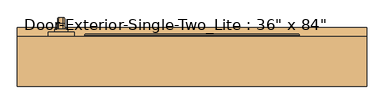
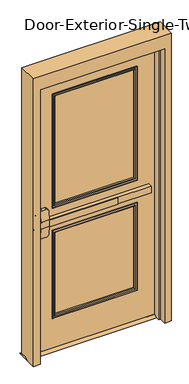
"""IFC4 building model written with IfcOpenShell, lengths in millimetres: door geometry."""

from ifc_helpers import new_model, si_unit, point, frame, frame_2d, origin, place, context, project, spatial, polyline, circle_curve, ellipse_curve, trimmed, segment, composite_curve, outline, extrude, faceted_brep, source, transform, mapped, element, save
from ifc_brep_helpers import plane_surface, cylinder_surface, revolved_surface, advanced_brep


def door_1117bd37(model_context):
    return source(origin(), model_context, "Body", "SolidModel", [
        extrude(outline(polyline([(76.2, 12.7), (120.65, 12.7), (146.05, 0.0), (50.8, 0.0), (76.2, 12.7)])), frame((-508.0, 0.0, 0.0), z_axis=(1.0, 0.0, 0.0), x_axis=(0.0, 1.0, 0.0)), (0.0, 0.0, 1.0), 1016.0),
        extrude(outline(polyline([(150.2833333, 38.1), (-349.25, 38.1), (-349.25, 44.45), (150.2833333, 44.45), (150.2833333, 38.1)])), frame((0.0, 0.0, 990.6), z_axis=(0.0, 0.0, 1.0), x_axis=(1.0, 0.0, 0.0)), (0.0, 0.0, 1.0), 50.8),
        advanced_brep(
        [(-412.75, 44.45, 1041.4), (-412.75, 44.45, 990.6), (-349.25, 44.45, 990.6), (400.05, 44.45, 990.6), (400.05, 44.45, 1041.4), (-349.25, 44.45, 1041.4), (400.05, 76.2, 1041.4), (400.05, 76.2, 990.6), (-349.25, 76.2, 990.6), (-349.25, 76.2, 927.1), (-368.3, 76.2, 908.05), (-393.7, 76.2, 908.05), (-412.75, 76.2, 927.1), (-412.75, 76.2, 1104.9), (-393.7, 76.2, 1123.95), (-368.3, 76.2, 1123.95), (-349.25, 76.2, 1104.9), (-349.25, 76.2, 1041.4), (-349.25, 47.6252467, 1041.4), (-412.75, 47.6252467, 1041.4), (-412.75, 52.6354269, 1104.9), (-412.75, 52.6354269, 927.1), (-412.75, 47.6252467, 990.6), (-349.25, 47.6252467, 990.6), (-349.25, 52.6354269, 927.1), (-349.25, 52.6354269, 1104.9), (-393.7, 54.138481, 1123.95), (-368.3, 54.138481, 1123.95), (-368.3, 54.138481, 908.05), (-393.7, 54.138481, 908.05)],
        [
            (0, 1),
            (1, 2),
            (2, 3),
            (3, 4),
            (4, 5),
            (5, 0),
            (6, 7),
            (7, 8),
            (8, 9),
            (9, 10, circle_curve(frame((-368.3, 76.2, 927.1), z_axis=(0.0, 1.0, 0.0), x_axis=(1.0, 0.0, 0.0)), 19.05)),
            (10, 11),
            (11, 12, circle_curve(frame((-393.7, 76.2, 927.1), z_axis=(0.0, 1.0, 0.0), x_axis=(1.0, 0.0, 0.0)), 19.05)),
            (12, 13),
            (13, 14, circle_curve(frame((-393.7, 76.2, 1104.9), z_axis=(0.0, 1.0, 0.0), x_axis=(1.0, 0.0, 0.0)), 19.05)),
            (14, 15),
            (15, 16, circle_curve(frame((-368.3, 76.2, 1104.9), z_axis=(0.0, 1.0, 0.0), x_axis=(1.0, 0.0, 0.0)), 19.05)),
            (16, 17),
            (17, 6),
            (4, 6),
            (17, 18),
            (18, 19),
            (19, 0),
            (19, 20),
            (20, 13),
            (12, 21),
            (21, 22),
            (22, 1),
            (7, 3),
            (22, 23),
            (23, 8),
            (23, 24),
            (24, 9),
            (16, 25),
            (25, 18),
            (14, 26),
            (26, 27),
            (27, 15),
            (10, 28),
            (28, 29),
            (29, 11),
            (24, 28, ellipse_curve(frame((-368.3, 52.6354269, 927.1), z_axis=(0.0, 0.9969018152893365, 0.07865602756830282), x_axis=(0.0, -0.07865602756830208, 0.9969018152893365)), 19.1092038, 19.05)),
            (27, 25, ellipse_curve(frame((-368.3, 52.6354269, 1104.9), z_axis=(0.0, 0.9969018152893376, -0.07865602756828934), x_axis=(0.0, -0.078656027568288, -0.9969018152893377)), 19.1092038, 19.05)),
            (20, 26, ellipse_curve(frame((-393.7, 52.6354269, 1104.9), z_axis=(0.0, 0.9969018152893376, -0.07865602756828934), x_axis=(0.0, -0.078656027568288, -0.9969018152893377)), 19.1092038, 19.05)),
            (29, 21, ellipse_curve(frame((-393.7, 52.6354269, 927.1), z_axis=(0.0, 0.9969018152893365, 0.07865602756830282), x_axis=(0.0, -0.07865602756830208, 0.9969018152893365)), 19.1092038, 19.05)),
        ],
        [
            plane_surface(frame((-412.75, 44.45, 1041.4), z_axis=(0.0, -1.0, 0.0), x_axis=(-1.0, 0.0, 0.0))),
            plane_surface(frame((-412.75, 76.2, 1041.4), z_axis=(0.0, 1.0, 0.0), x_axis=(1.0, 0.0, 0.0))),
            plane_surface(frame((400.05, 44.45, 1041.4), z_axis=(0.0, 0.0, 1.0), x_axis=(0.0, 1.0, 0.0))),
            plane_surface(frame((-412.75, 44.45, 1041.4), z_axis=(-1.0, 0.0, 0.0), x_axis=(0.0, 1.0, 0.0))),
            plane_surface(frame((-412.75, 44.45, 990.6), z_axis=(0.0, 0.0, -1.0), x_axis=(0.0, 1.0, 0.0))),
            plane_surface(frame((400.05, 44.45, 990.6), z_axis=(1.0, 0.0, 0.0), x_axis=(0.0, 1.0, 0.0))),
            plane_surface(frame((-349.25, 47.6252467, 927.1), z_axis=(1.0, 0.0, 0.0), x_axis=(0.0, 1.0, 0.0))),
            plane_surface(frame((-368.3, 47.6252467, 1123.95), z_axis=(0.0, 0.0, 1.0), x_axis=(0.0, 1.0, 0.0))),
            plane_surface(frame((-393.7, 47.6252467, 908.05), z_axis=(0.0, 0.0, -1.0), x_axis=(0.0, 1.0, 0.0))),
            cylinder_surface(frame((-368.3, 76.2, 927.1), z_axis=(0.0, -1.0, 0.0), x_axis=(1.0, 0.0, 0.0)), 19.05),
            cylinder_surface(frame((-368.3, 76.2, 1104.9), z_axis=(0.0, -1.0, 0.0), x_axis=(1.0, 0.0, 0.0)), 19.05),
            cylinder_surface(frame((-393.7, 76.2, 1104.9), z_axis=(0.0, -1.0, 0.0), x_axis=(1.0, 0.0, 0.0)), 19.05),
            cylinder_surface(frame((-393.7, 76.2, 927.1), z_axis=(0.0, -1.0, 0.0), x_axis=(1.0, 0.0, 0.0)), 19.05),
            plane_surface(frame((-349.25, 47.6252467, 1041.4), z_axis=(0.0, -0.9969018152893376, 0.07865602756828934), x_axis=(-1.0, 0.0, 0.0))),
            plane_surface(frame((-349.25, 54.138481, 908.05), z_axis=(0.0, -0.9969018152893365, -0.07865602756830282), x_axis=(-1.0, 0.0, 0.0))),
        ],
        [
            (0, [[1, 2, 3, 4, 5, 6]]),
            (1, [[7, 8, 9, 10, 11, 12, 13, 14, 15, 16, 17, 18]]),
            (2, [[19, -18, 20, 21, 22, -6, -5]]),
            (3, [[-1, -22, 23, 24, -13, 25, 26, 27]]),
            (4, [[28, -3, -2, -27, 29, 30, -8]]),
            (5, [[-4, -28, -7, -19]]),
            (6, [[-9, -30, 31, 32]]),
            (6, [[-17, 33, 34, -20]]),
            (7, [[-15, 35, 36, 37]]),
            (8, [[-11, 38, 39, 40]]),
            (9, [[-10, -32, 41, -38]]),
            (10, [[-16, -37, 42, -33]]),
            (11, [[-14, -24, 43, -35]]),
            (12, [[-12, -40, 44, -25]]),
            (13, [[-21, -34, -42, -36, -43, -23]]),
            (14, [[-26, -44, -39, -41, -31, -29]]),
        ],
    ),
        advanced_brep(
        [(-391.0, 133.35, 1017.190625), (-391.0, 133.35, 1014.809375), (-387.428125, 133.35, 1011.2375), (-374.5715406, 133.35, 1011.2375), (-371.0, 133.35, 1014.8090406), (-371.0, 133.35, 1017.190625), (-374.571875, 133.35, 1020.7625), (-387.428125, 133.35, 1020.7625), (-391.0, 133.35, 887.809375), (-387.428125, 133.35, 884.2375), (-374.571875, 133.35, 884.2375), (-371.0, 133.35, 887.809375), (-371.0, 133.35, 890.1909594), (-374.5715406, 133.35, 893.7625), (-387.428125, 133.35, 893.7625), (-391.0, 133.35, 890.190625), (-391.0, 158.75, 1017.190625), (-391.0, 172.640625, 1003.3), (-391.0, 172.640625, 901.7), (-391.0, 158.75, 887.809375), (-391.0, 158.75, 890.190625), (-391.0, 170.259375, 901.7), (-391.0, 170.259375, 1003.3), (-391.0, 158.75, 1014.809375), (-387.428125, 158.75, 1011.2375), (-374.5715406, 158.75, 1011.2375), (-371.0, 158.75, 1014.8090406), (-371.0, 170.2590406, 1003.3), (-371.0, 170.2590406, 901.7), (-371.0, 158.75, 890.1909594), (-371.0, 158.75, 887.809375), (-371.0, 172.640625, 901.7), (-371.0, 172.640625, 1003.3), (-371.0, 158.75, 1017.190625), (-374.571875, 158.75, 1020.7625), (-387.428125, 158.75, 1020.7625), (-387.428125, 166.6875, 1003.3), (-374.5715406, 166.6875, 1003.3), (-374.571875, 176.2125, 1003.3), (-387.428125, 176.2125, 1003.3), (-387.428125, 166.6875, 901.7), (-374.5715406, 166.6875, 901.7), (-374.571875, 176.2125, 901.7), (-387.428125, 176.2125, 901.7), (-387.428125, 158.75, 893.7625), (-374.5715406, 158.75, 893.7625), (-374.571875, 158.75, 884.2375), (-387.428125, 158.75, 884.2375)],
        [
            (0, 1),
            (1, 2, circle_curve(frame((-387.428125, 133.35, 1014.809375), z_axis=(0.0, -1.0, 0.0), x_axis=(0.0, 0.0, 1.0)), 3.571875)),
            (2, 3),
            (3, 4, circle_curve(frame((-374.5715406, 133.35, 1014.8090406), z_axis=(0.0, -1.0, 0.0), x_axis=(0.0, 0.0, 1.0)), 3.5715406)),
            (4, 5),
            (5, 6, circle_curve(frame((-374.571875, 133.35, 1017.190625), z_axis=(0.0, -1.0, 0.0), x_axis=(0.0, 0.0, 1.0)), 3.571875)),
            (6, 7),
            (7, 0, circle_curve(frame((-387.428125, 133.35, 1017.190625), z_axis=(0.0, -1.0, 0.0), x_axis=(0.0, 0.0, 1.0)), 3.571875)),
            (8, 9, circle_curve(frame((-387.428125, 133.35, 887.809375), z_axis=(0.0, -1.0, 0.0), x_axis=(0.0, 0.0, -1.0)), 3.571875)),
            (9, 10),
            (10, 11, circle_curve(frame((-374.571875, 133.35, 887.809375), z_axis=(0.0, -1.0, 0.0), x_axis=(0.0, 0.0, -1.0)), 3.571875)),
            (11, 12),
            (12, 13, circle_curve(frame((-374.5715406, 133.35, 890.1909594), z_axis=(0.0, -1.0, 0.0), x_axis=(0.0, 0.0, -1.0)), 3.5715406)),
            (13, 14),
            (14, 15, circle_curve(frame((-387.428125, 133.35, 890.190625), z_axis=(0.0, -1.0, 0.0), x_axis=(0.0, 0.0, -1.0)), 3.571875)),
            (15, 8),
            (0, 16),
            (16, 17, circle_curve(frame((-391.0, 158.75, 1003.3), z_axis=(-1.0, 0.0, 0.0), x_axis=(0.0, 0.0, 1.0)), 13.890625)),
            (17, 18),
            (18, 19, circle_curve(frame((-391.0, 158.75, 901.7), z_axis=(-1.0, 0.0, 0.0), x_axis=(0.0, 1.0, 0.0)), 13.890625)),
            (19, 8),
            (15, 20),
            (20, 21, circle_curve(frame((-391.0, 158.75, 901.7), z_axis=(1.0, 0.0, 0.0), x_axis=(0.0, 1.0, 0.0)), 11.509375)),
            (21, 22),
            (22, 23, circle_curve(frame((-391.0, 158.75, 1003.3), z_axis=(1.0, 0.0, 0.0), x_axis=(0.0, 0.0, 1.0)), 11.509375)),
            (23, 1),
            (23, 24, circle_curve(frame((-387.428125, 158.75, 1014.809375), z_axis=(0.0, -1.0, 0.0), x_axis=(0.0, 0.0, 1.0)), 3.571875)),
            (24, 2),
            (24, 25),
            (25, 3),
            (25, 26, circle_curve(frame((-374.5715406, 158.75, 1014.8090406), z_axis=(0.0, -1.0, 0.0), x_axis=(0.0, 0.0, 1.0)), 3.5715406)),
            (26, 4),
            (26, 27, circle_curve(frame((-371.0, 158.75, 1003.3), z_axis=(-1.0, 0.0, 0.0), x_axis=(0.0, 0.0, 1.0)), 11.5090406)),
            (27, 28),
            (28, 29, circle_curve(frame((-371.0, 158.75, 901.7), z_axis=(-1.0, 0.0, 0.0), x_axis=(0.0, 1.0, 0.0)), 11.5090406)),
            (29, 12),
            (11, 30),
            (30, 31, circle_curve(frame((-371.0, 158.75, 901.7), z_axis=(1.0, 0.0, 0.0), x_axis=(0.0, 1.0, 0.0)), 13.890625)),
            (31, 32),
            (32, 33, circle_curve(frame((-371.0, 158.75, 1003.3), z_axis=(1.0, 0.0, 0.0), x_axis=(0.0, 0.0, 1.0)), 13.890625)),
            (33, 5),
            (33, 34, circle_curve(frame((-374.571875, 158.75, 1017.190625), z_axis=(0.0, -1.0, 0.0), x_axis=(0.0, 0.0, 1.0)), 3.571875)),
            (34, 6),
            (34, 35),
            (35, 7),
            (35, 16, circle_curve(frame((-387.428125, 158.75, 1017.190625), z_axis=(0.0, -1.0, 0.0), x_axis=(0.0, 0.0, 1.0)), 3.571875)),
            (36, 24, circle_curve(frame((-387.428125, 158.75, 1003.3), z_axis=(1.0, 0.0, 0.0), x_axis=(0.0, 0.0, 1.0)), 7.9375)),
            (22, 36, circle_curve(frame((-387.428125, 170.259375, 1003.3), z_axis=(0.0, 0.0, 1.0), x_axis=(0.0, 1.0, 0.0)), 3.571875)),
            (37, 25, circle_curve(frame((-374.5715406, 158.75, 1003.3), z_axis=(1.0, 0.0, 0.0), x_axis=(0.0, 0.0, 1.0)), 7.9375)),
            (36, 37),
            (37, 27, circle_curve(frame((-374.5715406, 170.2590406, 1003.3), z_axis=(0.0, 0.0, 1.0), x_axis=(0.0, 1.0, 0.0)), 3.5715406)),
            (38, 34, circle_curve(frame((-374.571875, 158.75, 1003.3), z_axis=(1.0, 0.0, 0.0), x_axis=(0.0, 0.0, 1.0)), 17.4625)),
            (32, 38, circle_curve(frame((-374.571875, 172.640625, 1003.3), z_axis=(0.0, 0.0, 1.0), x_axis=(0.0, 1.0, 0.0)), 3.571875)),
            (39, 35, circle_curve(frame((-387.428125, 158.75, 1003.3), z_axis=(1.0, 0.0, 0.0), x_axis=(0.0, 0.0, 1.0)), 17.4625)),
            (38, 39),
            (39, 17, circle_curve(frame((-387.428125, 172.640625, 1003.3), z_axis=(0.0, 0.0, 1.0), x_axis=(0.0, 1.0, 0.0)), 3.571875)),
            (21, 40, circle_curve(frame((-387.428125, 170.259375, 901.7), z_axis=(0.0, 0.0, 1.0), x_axis=(0.0, 1.0, 0.0)), 3.571875)),
            (40, 36),
            (40, 41),
            (41, 37),
            (41, 28, circle_curve(frame((-374.5715406, 170.2590406, 901.7), z_axis=(0.0, 0.0, 1.0), x_axis=(0.0, 1.0, 0.0)), 3.5715406)),
            (31, 42, circle_curve(frame((-374.571875, 172.640625, 901.7), z_axis=(0.0, 0.0, 1.0), x_axis=(0.0, 1.0, 0.0)), 3.571875)),
            (42, 38),
            (42, 43),
            (43, 39),
            (43, 18, circle_curve(frame((-387.428125, 172.640625, 901.7), z_axis=(0.0, 0.0, 1.0), x_axis=(0.0, 1.0, 0.0)), 3.571875)),
            (44, 40, circle_curve(frame((-387.428125, 158.75, 901.7), z_axis=(1.0, 0.0, 0.0), x_axis=(0.0, 1.0, 0.0)), 7.9375)),
            (20, 44, circle_curve(frame((-387.428125, 158.75, 890.190625), z_axis=(0.0, 1.0, 0.0), x_axis=(0.0, 0.0, -1.0)), 3.571875)),
            (45, 41, circle_curve(frame((-374.5715406, 158.75, 901.7), z_axis=(1.0, 0.0, 0.0), x_axis=(0.0, 1.0, 0.0)), 7.9375)),
            (44, 45),
            (45, 29, circle_curve(frame((-374.5715406, 158.75, 890.1909594), z_axis=(0.0, 1.0, 0.0), x_axis=(0.0, 0.0, -1.0)), 3.5715406)),
            (46, 42, circle_curve(frame((-374.571875, 158.75, 901.7), z_axis=(1.0, 0.0, 0.0), x_axis=(0.0, 1.0, 0.0)), 17.4625)),
            (30, 46, circle_curve(frame((-374.571875, 158.75, 887.809375), z_axis=(0.0, 1.0, 0.0), x_axis=(0.0, 0.0, -1.0)), 3.571875)),
            (47, 43, circle_curve(frame((-387.428125, 158.75, 901.7), z_axis=(1.0, 0.0, 0.0), x_axis=(0.0, 1.0, 0.0)), 17.4625)),
            (46, 47),
            (47, 19, circle_curve(frame((-387.428125, 158.75, 887.809375), z_axis=(0.0, 1.0, 0.0), x_axis=(0.0, 0.0, -1.0)), 3.571875)),
            (14, 44),
            (13, 45),
            (10, 46),
            (9, 47),
        ],
        [
            plane_surface(frame((-381.0, 133.35, 1016.0), z_axis=(0.0, -1.0, 0.0), x_axis=(1.0, 0.0, 0.0))),
            plane_surface(frame((-381.0, 133.35, 889.0), z_axis=(0.0, -1.0, 0.0), x_axis=(1.0, 0.0, 0.0))),
            plane_surface(frame((-391.0, 133.35, 1017.190625), z_axis=(-1.0, 0.0, 0.0), x_axis=(0.0, 1.0, 0.0))),
            cylinder_surface(frame((-387.428125, 133.35, 1014.809375), z_axis=(0.0, -1.0, 0.0), x_axis=(0.0, 0.0, 1.0)), 3.571875),
            plane_surface(frame((-387.428125, 133.35, 1011.2375), z_axis=(0.0, 0.0, -1.0), x_axis=(0.0, 1.0, 0.0))),
            cylinder_surface(frame((-374.5715406, 133.35, 1014.8090406), z_axis=(0.0, -1.0, 0.0), x_axis=(0.0, 0.0, 1.0)), 3.5715406),
            plane_surface(frame((-371.0, 133.35, 1014.8090406), z_axis=(1.0, 0.0, 0.0), x_axis=(0.0, 1.0, 0.0))),
            cylinder_surface(frame((-374.571875, 133.35, 1017.190625), z_axis=(0.0, -1.0, 0.0), x_axis=(0.0, 0.0, 1.0)), 3.571875),
            plane_surface(frame((-374.571875, 133.35, 1020.7625), z_axis=(0.0, 0.0, 1.0), x_axis=(0.0, 1.0, 0.0))),
            cylinder_surface(frame((-387.428125, 133.35, 1017.190625), z_axis=(0.0, -1.0, 0.0), x_axis=(0.0, 0.0, 1.0)), 3.571875),
            revolved_surface(trimmed(ellipse_curve(frame((-387.428125, 158.75, 1014.809375), z_axis=(0.0, -1.0, 0.0), x_axis=(0.0, 0.0, 1.0)), 3.571875, 3.571875), [point((-391.0, 158.75, 1014.809375))], [point((-387.428125, 158.75, 1011.2375))], True, "CARTESIAN"), (-381.0, 158.75, 1003.3), (-1.0, 0.0, 0.0)),
            revolved_surface(polyline([(-387.428125, 158.75, 1011.2375), (-374.5715406, 158.75, 1011.2375)]), (-381.0, 158.75, 1003.3), (-1.0, 0.0, 0.0)),
            revolved_surface(trimmed(ellipse_curve(frame((-374.5715406, 158.75, 1014.8090406), z_axis=(0.0, -1.0, 0.0), x_axis=(0.0, 0.0, 1.0)), 3.5715406, 3.5715406), [point((-374.5715406, 158.75, 1011.2375))], [point((-371.0, 158.75, 1014.8090406))], True, "CARTESIAN"), (-381.0, 158.75, 1003.3), (-1.0, 0.0, 0.0)),
            revolved_surface(trimmed(ellipse_curve(frame((-374.571875, 158.75, 1017.190625), z_axis=(0.0, -1.0, 0.0), x_axis=(0.0, 0.0, 1.0)), 3.571875, 3.571875), [point((-371.0, 158.75, 1017.190625))], [point((-374.571875, 158.75, 1020.7625))], True, "CARTESIAN"), (-381.0, 158.75, 1003.3), (-1.0, 0.0, 0.0)),
            cylinder_surface(frame((-381.0, 158.75, 1003.3), z_axis=(-1.0, 0.0, 0.0), x_axis=(0.0, 0.0, 1.0)), 17.4625),
            revolved_surface(trimmed(ellipse_curve(frame((-387.428125, 158.75, 1017.190625), z_axis=(0.0, -1.0, 0.0), x_axis=(0.0, 0.0, 1.0)), 3.571875, 3.571875), [point((-387.428125, 158.75, 1020.7625))], [point((-391.0, 158.75, 1017.190625))], True, "CARTESIAN"), (-381.0, 158.75, 1003.3), (-1.0, 0.0, 0.0)),
            cylinder_surface(frame((-387.428125, 170.259375, 1003.3), z_axis=(0.0, 0.0, 1.0), x_axis=(0.0, 1.0, 0.0)), 3.571875),
            plane_surface(frame((-387.428125, 166.6875, 1003.3), z_axis=(0.0, -1.0, 0.0), x_axis=(0.0, 0.0, -1.0))),
            cylinder_surface(frame((-374.5715406, 170.2590406, 1003.3), z_axis=(0.0, 0.0, 1.0), x_axis=(0.0, 1.0, 0.0)), 3.5715406),
            cylinder_surface(frame((-374.571875, 172.640625, 1003.3), z_axis=(0.0, 0.0, 1.0), x_axis=(0.0, 1.0, 0.0)), 3.571875),
            plane_surface(frame((-374.571875, 176.2125, 1003.3), z_axis=(0.0, 1.0, 0.0), x_axis=(0.0, 0.0, -1.0))),
            cylinder_surface(frame((-387.428125, 172.640625, 1003.3), z_axis=(0.0, 0.0, 1.0), x_axis=(0.0, 1.0, 0.0)), 3.571875),
            revolved_surface(trimmed(ellipse_curve(frame((-387.428125, 170.259375, 901.7), z_axis=(0.0, 0.0, 1.0), x_axis=(0.0, 1.0, 0.0)), 3.571875, 3.571875), [point((-391.0, 170.259375, 901.7))], [point((-387.428125, 166.6875, 901.7))], True, "CARTESIAN"), (-381.0, 158.75, 901.7), (-1.0, 0.0, 0.0)),
            revolved_surface(polyline([(-387.428125, 166.6875, 901.7), (-374.5715406, 166.6875, 901.7)]), (-381.0, 158.75, 901.7), (-1.0, 0.0, 0.0)),
            revolved_surface(trimmed(ellipse_curve(frame((-374.5715406, 170.2590406, 901.7), z_axis=(0.0, 0.0, 1.0), x_axis=(0.0, 1.0, 0.0)), 3.5715406, 3.5715406), [point((-374.5715406, 166.6875, 901.7))], [point((-371.0, 170.2590406, 901.7))], True, "CARTESIAN"), (-381.0, 158.75, 901.7), (-1.0, 0.0, 0.0)),
            revolved_surface(trimmed(ellipse_curve(frame((-374.571875, 172.640625, 901.7), z_axis=(0.0, 0.0, 1.0), x_axis=(0.0, 1.0, 0.0)), 3.571875, 3.571875), [point((-371.0, 172.640625, 901.7))], [point((-374.571875, 176.2125, 901.7))], True, "CARTESIAN"), (-381.0, 158.75, 901.7), (-1.0, 0.0, 0.0)),
            cylinder_surface(frame((-381.0, 158.75, 901.7), z_axis=(-1.0, 0.0, 0.0), x_axis=(0.0, 1.0, 0.0)), 17.4625),
            revolved_surface(trimmed(ellipse_curve(frame((-387.428125, 172.640625, 901.7), z_axis=(0.0, 0.0, 1.0), x_axis=(0.0, 1.0, 0.0)), 3.571875, 3.571875), [point((-387.428125, 176.2125, 901.7))], [point((-391.0, 172.640625, 901.7))], True, "CARTESIAN"), (-381.0, 158.75, 901.7), (-1.0, 0.0, 0.0)),
            cylinder_surface(frame((-387.428125, 158.75, 890.190625), z_axis=(0.0, 1.0, 0.0), x_axis=(0.0, 0.0, -1.0)), 3.571875),
            plane_surface(frame((-387.428125, 158.75, 893.7625), z_axis=(0.0, 0.0, 1.0), x_axis=(0.0, -1.0, 0.0))),
            cylinder_surface(frame((-374.5715406, 158.75, 890.1909594), z_axis=(0.0, 1.0, 0.0), x_axis=(0.0, 0.0, -1.0)), 3.5715406),
            cylinder_surface(frame((-374.571875, 158.75, 887.809375), z_axis=(0.0, 1.0, 0.0), x_axis=(0.0, 0.0, -1.0)), 3.571875),
            plane_surface(frame((-374.571875, 158.75, 884.2375), z_axis=(0.0, 0.0, -1.0), x_axis=(0.0, -1.0, 0.0))),
            cylinder_surface(frame((-387.428125, 158.75, 887.809375), z_axis=(0.0, 1.0, 0.0), x_axis=(0.0, 0.0, -1.0)), 3.571875),
        ],
        [
            (0, [[1, 2, 3, 4, 5, 6, 7, 8]]),
            (1, [[9, 10, 11, 12, 13, 14, 15, 16]]),
            (2, [[-1, 17, 18, 19, 20, 21, -16, 22, 23, 24, 25, 26]]),
            (3, [[-2, -26, 27, 28]]),
            (4, [[-3, -28, 29, 30]]),
            (5, [[-4, -30, 31, 32]]),
            (6, [[-5, -32, 33, 34, 35, 36, -12, 37, 38, 39, 40, 41]]),
            (7, [[-6, -41, 42, 43]]),
            (8, [[-7, -43, 44, 45]]),
            (9, [[-8, -45, 46, -17]]),
            (10, [[47, -27, -25, 48]]),
            (11, [[49, -29, -47, 50]]),
            (12, [[-33, -31, -49, 51]]),
            (13, [[52, -42, -40, 53]]),
            (14, [[54, -44, -52, 55]]),
            (15, [[-18, -46, -54, 56]]),
            (16, [[-48, -24, 57, 58]]),
            (17, [[-50, -58, 59, 60]]),
            (18, [[-51, -60, 61, -34]]),
            (19, [[-53, -39, 62, 63]]),
            (20, [[-55, -63, 64, 65]]),
            (21, [[-56, -65, 66, -19]]),
            (22, [[67, -57, -23, 68]]),
            (23, [[69, -59, -67, 70]]),
            (24, [[-35, -61, -69, 71]]),
            (25, [[72, -62, -38, 73]]),
            (26, [[74, -64, -72, 75]]),
            (27, [[-20, -66, -74, 76]]),
            (28, [[-68, -22, -15, 77]]),
            (29, [[-70, -77, -14, 78]]),
            (30, [[-71, -78, -13, -36]]),
            (31, [[-73, -37, -11, 79]]),
            (32, [[-75, -79, -10, 80]]),
            (33, [[-76, -80, -9, -21]]),
        ],
    ),
        extrude(outline(composite_curve([segment(trimmed(circle_curve(frame_2d((1117.6, -381.0)), 19.0), [point((1117.6, -400.0))], [point((1117.6, -362.0))], False, "CARTESIAN"), True, "CONTINUOUS"), segment(trimmed(circle_curve(frame_2d((1117.6, -381.0)), 19.0), [point((1117.6, -362.0))], [point((1117.6, -400.0))], False, "CARTESIAN"), True, "CONTINUOUS")], self_intersect=False)), frame((0.0, 133.35, 0.0), z_axis=(0.0, 1.0, 0.0), x_axis=(0.0, 0.0, 1.0)), (0.0, 0.0, 1.0), 8.73125),
        extrude(outline(composite_curve([segment(trimmed(circle_curve(frame_2d((1113.0338574, -381.0)), 89.3016225), [point((1193.8, -342.9))], [point((1193.8, -419.1))], False, "CARTESIAN"), True, "CONTINUOUS"), segment(polyline([(1193.8, -419.1), (838.2, -419.1)]), True, "CONTINUOUS"), segment(trimmed(circle_curve(frame_2d((918.9661426, -381.0)), 89.3016225), [point((838.2, -419.1))], [point((838.2, -342.9))], False, "CARTESIAN"), True, "CONTINUOUS"), segment(polyline([(838.2, -342.9), (1193.8, -342.9)]), True, "CONTINUOUS")], self_intersect=False)), frame((0.0, 120.65, 0.0), z_axis=(0.0, 1.0, 0.0), x_axis=(0.0, 0.0, 1.0)), (0.0, 0.0, 1.0), 12.7),
        faceted_brep([(457.2, 71.4375, 0.0), (457.2, 120.65, 0.0), (508.0, 120.65, 0.0), (508.0, -25.4, 0.0), (457.2, -25.4, 0.0), (457.2, 23.8125, 0.0), (441.325, 23.8125, 0.0), (441.325, 71.4375, 0.0), (457.2, 71.4375, 2133.6), (457.2, 120.65, 2133.6), (-457.2, 120.65, 2133.6), (-457.2, 120.65, 0.0), (-508.0, 120.65, 0.0), (-508.0, 120.65, 2235.2), (508.0, 120.65, 2235.2), (508.0, -25.4, 2235.2), (-508.0, -25.4, 2235.2), (-508.0, -25.4, 0.0), (-457.2, -25.4, 0.0), (-457.2, -25.4, 2133.6), (457.2, -25.4, 2133.6), (457.2, 23.8125, 2133.6), (-457.2, 23.8125, 2133.6), (-457.2, 23.8125, 0.0), (-441.325, 23.8125, 0.0), (-441.325, 23.8125, 2117.725), (441.325, 23.8125, 2117.725), (441.325, 71.4375, 2117.725), (-441.325, 71.4375, 2117.725), (-441.325, 71.4375, 0.0), (-457.2, 71.4375, 0.0), (-457.2, 71.4375, 2133.6)], [[[0, 1, 2, 3, 4, 5, 6, 7]], [[1, 0, 8, 9]], [[2, 1, 9, 10, 11, 12, 13, 14]], [[3, 2, 14, 15]], [[4, 3, 15, 16, 17, 18, 19, 20]], [[5, 4, 20, 21]], [[6, 5, 21, 22, 23, 24, 25, 26]], [[7, 6, 26, 27]], [[0, 7, 27, 28, 29, 30, 31, 8]], [[9, 8, 31, 10]], [[20, 19, 22, 21]], [[26, 25, 28, 27]], [[12, 11, 30, 29, 24, 23, 18, 17]], [[11, 10, 31, 30]], [[13, 12, 17, 16]], [[19, 18, 23, 22]], [[25, 24, 29, 28]], [[15, 14, 13, 16]]]),
        extrude(outline(polyline([(2133.6, -457.2), (12.7, -457.2), (12.7, 457.2), (2133.6, 457.2), (2133.6, -457.2)]), holes=[polyline([(1981.2, -304.8), (1981.2, 304.8), (1111.25, 304.8), (1111.25, -304.8), (1981.2, -304.8)]), polyline([(920.75, -304.8), (920.75, 304.8), (254.0, 304.8), (254.0, -304.8), (920.75, -304.8)])]), frame((0.0, 76.2, 0.0), z_axis=(0.0, 1.0, 0.0), x_axis=(0.0, 0.0, 1.0)), (0.0, 0.0, 1.0), 44.45),
        extrude(outline(polyline([(304.8, 88.9), (-304.8, 88.9), (-304.8, 107.95), (304.8, 107.95), (304.8, 88.9)])), frame((0.0, 0.0, 1111.25), z_axis=(0.0, 0.0, 1.0), x_axis=(1.0, 0.0, 0.0)), (0.0, 0.0, 1.0), 869.95),
        extrude(outline(polyline([(304.8, 88.9), (-304.8, 88.9), (-304.8, 107.95), (304.8, 107.95), (304.8, 88.9)])), frame((0.0, 0.0, 254.0), z_axis=(0.0, 0.0, 1.0), x_axis=(1.0, 0.0, 0.0)), (0.0, 0.0, 1.0), 666.75),
        advanced_brep(
        [(304.8, 88.9, 920.75), (304.8, 76.2, 920.75), (304.8, 76.2, 254.0), (304.8, 88.9, 254.0), (292.8, 75.2, 908.75), (292.8, 88.9, 908.75), (292.8, 88.9, 266.0), (292.8, 75.2, 266.0), (297.8, 70.2, 913.75), (297.8, 70.2, 261.0), (312.8, 72.2, 928.75), (310.8, 70.2, 926.75), (310.8, 70.2, 248.0), (312.8, 72.2, 246.0), (312.8, 76.2, 928.75), (312.8, 76.2, 246.0), (-304.8, 76.2, 254.0), (-304.8, 88.9, 254.0), (-292.8, 88.9, 266.0), (-292.8, 75.2, 266.0), (-297.8, 70.2, 261.0), (-310.8, 70.2, 248.0), (-312.8, 72.2, 246.0), (-312.8, 76.2, 246.0), (-304.8, 76.2, 920.75), (-304.8, 88.9, 920.75), (-292.8, 88.9, 908.75), (-292.8, 75.2, 908.75), (-297.8, 70.2, 913.75), (-310.8, 70.2, 926.75), (-312.8, 72.2, 928.75), (-312.8, 76.2, 928.75)],
        [
            (0, 1),
            (1, 2),
            (2, 3),
            (3, 0),
            (4, 5),
            (5, 6),
            (6, 7),
            (7, 4),
            (8, 4, ellipse_curve(frame((297.8, 75.2, 913.75), z_axis=(0.7071067811865475, 0.0, -0.7071067811865475), x_axis=(0.7071067811865474, 0.0, 0.7071067811865476)), 7.0710678, 5.0)),
            (7, 9, ellipse_curve(frame((297.8, 75.2, 261.0), z_axis=(0.7071067811865475, 0.0, 0.7071067811865475), x_axis=(-0.7071067811865474, 0.0, 0.7071067811865476)), 7.0710678, 5.0)),
            (9, 8),
            (10, 11, ellipse_curve(frame((310.8, 72.2, 926.75), z_axis=(0.7071067811865475, 0.0, -0.7071067811865475), x_axis=(0.7071067811865474, 0.0, 0.7071067811865476)), 2.8284271, 2.0)),
            (11, 12),
            (12, 13, ellipse_curve(frame((310.8, 72.2, 248.0), z_axis=(0.7071067811865475, 0.0, 0.7071067811865475), x_axis=(-0.7071067811865474, 0.0, 0.7071067811865476)), 2.8284271, 2.0)),
            (13, 10),
            (14, 10),
            (13, 15),
            (15, 14),
            (2, 16),
            (16, 17),
            (17, 3),
            (6, 18),
            (18, 19),
            (19, 7),
            (19, 20, ellipse_curve(frame((-297.8, 75.2, 261.0), z_axis=(0.7071067811865475, 0.0, -0.7071067811865475), x_axis=(0.7071067811865476, 0.0, 0.7071067811865474)), 7.0710678, 5.0)),
            (20, 9),
            (12, 21),
            (21, 22, ellipse_curve(frame((-310.8, 72.2, 248.0), z_axis=(0.7071067811865475, 0.0, -0.7071067811865475), x_axis=(0.7071067811865476, 0.0, 0.7071067811865474)), 2.8284271, 2.0)),
            (22, 13),
            (22, 23),
            (23, 15),
            (16, 24),
            (24, 25),
            (25, 17),
            (18, 26),
            (26, 27),
            (27, 19),
            (27, 28, ellipse_curve(frame((-297.8, 75.2, 913.75), z_axis=(-0.7071067811865475, 0.0, -0.7071067811865475), x_axis=(0.7071067811865474, 0.0, -0.7071067811865476)), 7.0710678, 5.0)),
            (28, 20),
            (21, 29),
            (29, 30, ellipse_curve(frame((-310.8, 72.2, 926.75), z_axis=(-0.7071067811865475, 0.0, -0.7071067811865475), x_axis=(0.7071067811865474, 0.0, -0.7071067811865476)), 2.8284271, 2.0)),
            (30, 22),
            (30, 31),
            (31, 23),
            (31, 14),
            (1, 24),
            (0, 25),
            (5, 26),
            (4, 27),
            (8, 28),
            (11, 29),
            (10, 30),
        ],
        [
            plane_surface(frame((304.8, 76.2, 920.75), z_axis=(1.0, 0.0, 0.0), x_axis=(0.0, 0.0, -1.0))),
            plane_surface(frame((292.8, 88.9, 908.75), z_axis=(-1.0, 0.0, 0.0), x_axis=(0.0, 0.0, -1.0))),
            cylinder_surface(frame((297.8, 75.2, 920.75), z_axis=(0.0, 0.0, 1.0), x_axis=(1.0, 0.0, 0.0)), 5.0),
            cylinder_surface(frame((310.8, 72.2, 920.75), z_axis=(0.0, 0.0, 1.0), x_axis=(1.0, 0.0, 0.0)), 2.0),
            plane_surface(frame((312.8, 72.2, 928.75), z_axis=(1.0, 0.0, 0.0), x_axis=(0.0, 0.0, -1.0))),
            plane_surface(frame((304.8, 76.2, 254.0), z_axis=(0.0, 0.0, -1.0), x_axis=(-1.0, 0.0, 0.0))),
            plane_surface(frame((292.8, 88.9, 266.0), z_axis=(0.0, 0.0, 1.0), x_axis=(-1.0, 0.0, 0.0))),
            cylinder_surface(frame((304.8, 75.2, 261.0), z_axis=(1.0, 0.0, 0.0), x_axis=(0.0, 0.0, -1.0)), 5.0),
            cylinder_surface(frame((304.8, 72.2, 248.0), z_axis=(1.0, 0.0, 0.0), x_axis=(0.0, 0.0, -1.0)), 2.0),
            plane_surface(frame((312.8, 72.2, 246.0), z_axis=(0.0, 0.0, -1.0), x_axis=(-1.0, 0.0, 0.0))),
            plane_surface(frame((-304.8, 76.2, 254.0), z_axis=(-1.0, 0.0, 0.0), x_axis=(0.0, 0.0, 1.0))),
            plane_surface(frame((-292.8, 88.9, 266.0), z_axis=(1.0, 0.0, 0.0), x_axis=(0.0, 0.0, 1.0))),
            cylinder_surface(frame((-297.8, 75.2, 254.0), z_axis=(0.0, 0.0, -1.0), x_axis=(-1.0, 0.0, 0.0)), 5.0),
            cylinder_surface(frame((-310.8, 72.2, 254.0), z_axis=(0.0, 0.0, -1.0), x_axis=(-1.0, 0.0, 0.0)), 2.0),
            plane_surface(frame((-312.8, 72.2, 246.0), z_axis=(-1.0, 0.0, 0.0), x_axis=(0.0, 0.0, 1.0))),
            plane_surface(frame((-312.8, 76.2, 928.75), z_axis=(0.0, 1.0, 0.0), x_axis=(1.0, 0.0, 0.0))),
            plane_surface(frame((-304.8, 76.2, 920.75), z_axis=(0.0, 0.0, 1.0), x_axis=(1.0, 0.0, 0.0))),
            plane_surface(frame((-304.8, 88.9, 920.75), z_axis=(0.0, 1.0, 0.0), x_axis=(1.0, 0.0, 0.0))),
            plane_surface(frame((-292.8, 88.9, 908.75), z_axis=(0.0, 0.0, -1.0), x_axis=(1.0, 0.0, 0.0))),
            cylinder_surface(frame((-304.8, 75.2, 913.75), z_axis=(-1.0, 0.0, 0.0), x_axis=(0.0, 0.0, 1.0)), 5.0),
            plane_surface(frame((-297.8, 70.2, 913.75), z_axis=(0.0, -1.0, 0.0), x_axis=(1.0, 0.0, 0.0))),
            cylinder_surface(frame((-304.8, 72.2, 926.75), z_axis=(-1.0, 0.0, 0.0), x_axis=(0.0, 0.0, 1.0)), 2.0),
            plane_surface(frame((-312.8, 72.2, 928.75), z_axis=(0.0, 0.0, 1.0), x_axis=(1.0, 0.0, 0.0))),
        ],
        [
            (0, [[1, 2, 3, 4]]),
            (1, [[5, 6, 7, 8]]),
            (2, [[9, -8, 10, 11]]),
            (3, [[12, 13, 14, 15]]),
            (4, [[16, -15, 17, 18]]),
            (5, [[-3, 19, 20, 21]]),
            (6, [[-7, 22, 23, 24]]),
            (7, [[-10, -24, 25, 26]]),
            (8, [[-14, 27, 28, 29]]),
            (9, [[-17, -29, 30, 31]]),
            (10, [[-20, 32, 33, 34]]),
            (11, [[-23, 35, 36, 37]]),
            (12, [[-25, -37, 38, 39]]),
            (13, [[-28, 40, 41, 42]]),
            (14, [[-30, -42, 43, 44]]),
            (15, [[-31, -44, 45, -18], [46, -32, -19, -2]]),
            (16, [[-33, -46, -1, 47]]),
            (17, [[-21, -34, -47, -4], [48, -35, -22, -6]]),
            (18, [[-36, -48, -5, 49]]),
            (19, [[-38, -49, -9, 50]]),
            (20, [[51, -40, -27, -13], [-26, -39, -50, -11]]),
            (21, [[-41, -51, -12, 52]]),
            (22, [[-43, -52, -16, -45]]),
        ],
    ),
        advanced_brep(
        [(-304.8, 107.95, 920.75), (-304.8, 120.65, 920.75), (-304.8, 120.65, 254.0), (-304.8, 107.95, 254.0), (-292.8, 121.65, 908.75), (-292.8, 107.95, 908.75), (-292.8, 107.95, 266.0), (-292.8, 121.65, 266.0), (-297.8, 126.65, 913.75), (-297.8, 126.65, 261.0), (-312.8, 124.65, 928.75), (-310.8, 126.65, 926.75), (-310.8, 126.65, 248.0), (-312.8, 124.65, 246.0), (-312.8, 120.65, 928.75), (-312.8, 120.65, 246.0), (304.8, 120.65, 254.0), (304.8, 107.95, 254.0), (292.8, 107.95, 266.0), (292.8, 121.65, 266.0), (297.8, 126.65, 261.0), (310.8, 126.65, 248.0), (312.8, 124.65, 246.0), (312.8, 120.65, 246.0), (304.8, 120.65, 920.75), (304.8, 107.95, 920.75), (292.8, 107.95, 908.75), (292.8, 121.65, 908.75), (297.8, 126.65, 913.75), (310.8, 126.65, 926.75), (312.8, 124.65, 928.75), (312.8, 120.65, 928.75)],
        [
            (0, 1),
            (1, 2),
            (2, 3),
            (3, 0),
            (4, 5),
            (5, 6),
            (6, 7),
            (7, 4),
            (8, 4, ellipse_curve(frame((-297.8, 121.65, 913.75), z_axis=(-0.7071067811865475, 0.0, -0.7071067811865475), x_axis=(-0.7071067811865474, 0.0, 0.7071067811865476)), 7.0710678, 5.0)),
            (7, 9, ellipse_curve(frame((-297.8, 121.65, 261.0), z_axis=(-0.7071067811865475, 0.0, 0.7071067811865475), x_axis=(0.7071067811865474, 0.0, 0.7071067811865476)), 7.0710678, 5.0)),
            (9, 8),
            (10, 11, ellipse_curve(frame((-310.8, 124.65, 926.75), z_axis=(-0.7071067811865475, 0.0, -0.7071067811865475), x_axis=(-0.7071067811865474, 0.0, 0.7071067811865476)), 2.8284271, 2.0)),
            (11, 12),
            (12, 13, ellipse_curve(frame((-310.8, 124.65, 248.0), z_axis=(-0.7071067811865475, 0.0, 0.7071067811865475), x_axis=(0.7071067811865474, 0.0, 0.7071067811865476)), 2.8284271, 2.0)),
            (13, 10),
            (14, 10),
            (13, 15),
            (15, 14),
            (2, 16),
            (16, 17),
            (17, 3),
            (6, 18),
            (18, 19),
            (19, 7),
            (19, 20, ellipse_curve(frame((297.8, 121.65, 261.0), z_axis=(-0.7071067811865475, 0.0, -0.7071067811865475), x_axis=(-0.7071067811865476, 0.0, 0.7071067811865474)), 7.0710678, 5.0)),
            (20, 9),
            (12, 21),
            (21, 22, ellipse_curve(frame((310.8, 124.65, 248.0), z_axis=(-0.7071067811865475, 0.0, -0.7071067811865475), x_axis=(-0.7071067811865476, 0.0, 0.7071067811865474)), 2.8284271, 2.0)),
            (22, 13),
            (22, 23),
            (23, 15),
            (16, 24),
            (24, 25),
            (25, 17),
            (18, 26),
            (26, 27),
            (27, 19),
            (27, 28, ellipse_curve(frame((297.8, 121.65, 913.75), z_axis=(0.7071067811865475, 0.0, -0.7071067811865475), x_axis=(-0.7071067811865474, 0.0, -0.7071067811865476)), 7.0710678, 5.0)),
            (28, 20),
            (21, 29),
            (29, 30, ellipse_curve(frame((310.8, 124.65, 926.75), z_axis=(0.7071067811865475, 0.0, -0.7071067811865475), x_axis=(-0.7071067811865474, 0.0, -0.7071067811865476)), 2.8284271, 2.0)),
            (30, 22),
            (30, 31),
            (31, 23),
            (31, 14),
            (1, 24),
            (0, 25),
            (5, 26),
            (4, 27),
            (8, 28),
            (11, 29),
            (10, 30),
        ],
        [
            plane_surface(frame((-304.8, 120.65, 920.75), z_axis=(-1.0, 0.0, 0.0), x_axis=(0.0, 0.0, -1.0))),
            plane_surface(frame((-292.8, 107.95, 908.75), z_axis=(1.0, 0.0, 0.0), x_axis=(0.0, 0.0, -1.0))),
            cylinder_surface(frame((-297.8, 121.65, 920.75), z_axis=(0.0, 0.0, 1.0), x_axis=(-1.0, 0.0, 0.0)), 5.0),
            cylinder_surface(frame((-310.8, 124.65, 920.75), z_axis=(0.0, 0.0, 1.0), x_axis=(-1.0, 0.0, 0.0)), 2.0),
            plane_surface(frame((-312.8, 124.65, 928.75), z_axis=(-1.0, 0.0, 0.0), x_axis=(0.0, 0.0, -1.0))),
            plane_surface(frame((-304.8, 120.65, 254.0), z_axis=(0.0, 0.0, -1.0), x_axis=(1.0, 0.0, 0.0))),
            plane_surface(frame((-292.8, 107.95, 266.0), z_axis=(0.0, 0.0, 1.0), x_axis=(1.0, 0.0, 0.0))),
            cylinder_surface(frame((-304.8, 121.65, 261.0), z_axis=(-1.0, 0.0, 0.0), x_axis=(0.0, 0.0, -1.0)), 5.0),
            cylinder_surface(frame((-304.8, 124.65, 248.0), z_axis=(-1.0, 0.0, 0.0), x_axis=(0.0, 0.0, -1.0)), 2.0),
            plane_surface(frame((-312.8, 124.65, 246.0), z_axis=(0.0, 0.0, -1.0), x_axis=(1.0, 0.0, 0.0))),
            plane_surface(frame((304.8, 120.65, 254.0), z_axis=(1.0, 0.0, 0.0), x_axis=(0.0, 0.0, 1.0))),
            plane_surface(frame((292.8, 107.95, 266.0), z_axis=(-1.0, 0.0, 0.0), x_axis=(0.0, 0.0, 1.0))),
            cylinder_surface(frame((297.8, 121.65, 254.0), z_axis=(0.0, 0.0, -1.0), x_axis=(1.0, 0.0, 0.0)), 5.0),
            cylinder_surface(frame((310.8, 124.65, 254.0), z_axis=(0.0, 0.0, -1.0), x_axis=(1.0, 0.0, 0.0)), 2.0),
            plane_surface(frame((312.8, 124.65, 246.0), z_axis=(1.0, 0.0, 0.0), x_axis=(0.0, 0.0, 1.0))),
            plane_surface(frame((312.8, 120.65, 928.75), z_axis=(0.0, -1.0, 0.0), x_axis=(-1.0, 0.0, 0.0))),
            plane_surface(frame((304.8, 120.65, 920.75), z_axis=(0.0, 0.0, 1.0), x_axis=(-1.0, 0.0, 0.0))),
            plane_surface(frame((304.8, 107.95, 920.75), z_axis=(0.0, -1.0, 0.0), x_axis=(-1.0, 0.0, 0.0))),
            plane_surface(frame((292.8, 107.95, 908.75), z_axis=(0.0, 0.0, -1.0), x_axis=(-1.0, 0.0, 0.0))),
            cylinder_surface(frame((304.8, 121.65, 913.75), z_axis=(1.0, 0.0, 0.0), x_axis=(0.0, 0.0, 1.0)), 5.0),
            plane_surface(frame((297.8, 126.65, 913.75), z_axis=(0.0, 1.0, 0.0), x_axis=(-1.0, 0.0, 0.0))),
            cylinder_surface(frame((304.8, 124.65, 926.75), z_axis=(1.0, 0.0, 0.0), x_axis=(0.0, 0.0, 1.0)), 2.0),
            plane_surface(frame((312.8, 124.65, 928.75), z_axis=(0.0, 0.0, 1.0), x_axis=(-1.0, 0.0, 0.0))),
        ],
        [
            (0, [[1, 2, 3, 4]]),
            (1, [[5, 6, 7, 8]]),
            (2, [[9, -8, 10, 11]]),
            (3, [[12, 13, 14, 15]]),
            (4, [[16, -15, 17, 18]]),
            (5, [[-3, 19, 20, 21]]),
            (6, [[-7, 22, 23, 24]]),
            (7, [[-10, -24, 25, 26]]),
            (8, [[-14, 27, 28, 29]]),
            (9, [[-17, -29, 30, 31]]),
            (10, [[-20, 32, 33, 34]]),
            (11, [[-23, 35, 36, 37]]),
            (12, [[-25, -37, 38, 39]]),
            (13, [[-28, 40, 41, 42]]),
            (14, [[-30, -42, 43, 44]]),
            (15, [[-31, -44, 45, -18], [46, -32, -19, -2]]),
            (16, [[-33, -46, -1, 47]]),
            (17, [[-21, -34, -47, -4], [48, -35, -22, -6]]),
            (18, [[-36, -48, -5, 49]]),
            (19, [[-38, -49, -9, 50]]),
            (20, [[51, -40, -27, -13], [-26, -39, -50, -11]]),
            (21, [[-41, -51, -12, 52]]),
            (22, [[-43, -52, -16, -45]]),
        ],
    ),
        advanced_brep(
        [(-304.8, 88.9, 1111.25), (-304.8, 76.2, 1111.25), (-304.8, 76.2, 1981.2), (-304.8, 88.9, 1981.2), (-292.8, 75.2, 1123.25), (-292.8, 88.9, 1123.25), (-292.8, 88.9, 1969.2), (-292.8, 75.2, 1969.2), (-297.8, 70.2, 1118.25), (-297.8, 70.2, 1974.2), (-312.8, 72.2, 1103.25), (-310.8, 70.2, 1105.25), (-310.8, 70.2, 1987.2), (-312.8, 72.2, 1989.2), (-312.8, 76.2, 1103.25), (-312.8, 76.2, 1989.2), (304.8, 76.2, 1981.2), (304.8, 88.9, 1981.2), (292.8, 88.9, 1969.2), (292.8, 75.2, 1969.2), (297.8, 70.2, 1974.2), (310.8, 70.2, 1987.2), (312.8, 72.2, 1989.2), (312.8, 76.2, 1989.2), (304.8, 76.2, 1111.25), (304.8, 88.9, 1111.25), (292.8, 88.9, 1123.25), (292.8, 75.2, 1123.25), (297.8, 70.2, 1118.25), (310.8, 70.2, 1105.25), (312.8, 72.2, 1103.25), (312.8, 76.2, 1103.25)],
        [
            (0, 1),
            (1, 2),
            (2, 3),
            (3, 0),
            (4, 5),
            (5, 6),
            (6, 7),
            (7, 4),
            (8, 4, ellipse_curve(frame((-297.8, 75.2, 1118.25), z_axis=(-0.7071067811865475, 0.0, 0.7071067811865475), x_axis=(-0.7071067811865474, 0.0, -0.7071067811865476)), 7.0710678, 5.0)),
            (7, 9, ellipse_curve(frame((-297.8, 75.2, 1974.2), z_axis=(-0.7071067811865475, 0.0, -0.7071067811865475), x_axis=(0.7071067811865474, 0.0, -0.7071067811865476)), 7.0710678, 5.0)),
            (9, 8),
            (10, 11, ellipse_curve(frame((-310.8, 72.2, 1105.25), z_axis=(-0.7071067811865475, 0.0, 0.7071067811865475), x_axis=(-0.7071067811865474, 0.0, -0.7071067811865476)), 2.8284271, 2.0)),
            (11, 12),
            (12, 13, ellipse_curve(frame((-310.8, 72.2, 1987.2), z_axis=(-0.7071067811865475, 0.0, -0.7071067811865475), x_axis=(0.7071067811865474, 0.0, -0.7071067811865476)), 2.8284271, 2.0)),
            (13, 10),
            (14, 10),
            (13, 15),
            (15, 14),
            (2, 16),
            (16, 17),
            (17, 3),
            (6, 18),
            (18, 19),
            (19, 7),
            (19, 20, ellipse_curve(frame((297.8, 75.2, 1974.2), z_axis=(-0.7071067811865475, 0.0, 0.7071067811865475), x_axis=(-0.7071067811865476, 0.0, -0.7071067811865474)), 7.0710678, 5.0)),
            (20, 9),
            (12, 21),
            (21, 22, ellipse_curve(frame((310.8, 72.2, 1987.2), z_axis=(-0.7071067811865475, 0.0, 0.7071067811865475), x_axis=(-0.7071067811865476, 0.0, -0.7071067811865474)), 2.8284271, 2.0)),
            (22, 13),
            (22, 23),
            (23, 15),
            (16, 24),
            (24, 25),
            (25, 17),
            (18, 26),
            (26, 27),
            (27, 19),
            (27, 28, ellipse_curve(frame((297.8, 75.2, 1118.25), z_axis=(0.7071067811865475, 0.0, 0.7071067811865475), x_axis=(-0.7071067811865474, 0.0, 0.7071067811865476)), 7.0710678, 5.0)),
            (28, 20),
            (21, 29),
            (29, 30, ellipse_curve(frame((310.8, 72.2, 1105.25), z_axis=(0.7071067811865475, 0.0, 0.7071067811865475), x_axis=(-0.7071067811865474, 0.0, 0.7071067811865476)), 2.8284271, 2.0)),
            (30, 22),
            (30, 31),
            (31, 23),
            (31, 14),
            (1, 24),
            (0, 25),
            (5, 26),
            (4, 27),
            (8, 28),
            (11, 29),
            (10, 30),
        ],
        [
            plane_surface(frame((-304.8, 76.2, 1111.25), z_axis=(-1.0, 0.0, 0.0), x_axis=(0.0, 0.0, 1.0))),
            plane_surface(frame((-292.8, 88.9, 1123.25), z_axis=(1.0, 0.0, 0.0), x_axis=(0.0, 0.0, 1.0))),
            cylinder_surface(frame((-297.8, 75.2, 1111.25), z_axis=(0.0, 0.0, -1.0), x_axis=(-1.0, 0.0, 0.0)), 5.0),
            cylinder_surface(frame((-310.8, 72.2, 1111.25), z_axis=(0.0, 0.0, -1.0), x_axis=(-1.0, 0.0, 0.0)), 2.0),
            plane_surface(frame((-312.8, 72.2, 1103.25), z_axis=(-1.0, 0.0, 0.0), x_axis=(0.0, 0.0, 1.0))),
            plane_surface(frame((-304.8, 76.2, 1981.2), z_axis=(0.0, 0.0, 1.0), x_axis=(1.0, 0.0, 0.0))),
            plane_surface(frame((-292.8, 88.9, 1969.2), z_axis=(0.0, 0.0, -1.0), x_axis=(1.0, 0.0, 0.0))),
            cylinder_surface(frame((-304.8, 75.2, 1974.2), z_axis=(-1.0, 0.0, 0.0), x_axis=(0.0, 0.0, 1.0)), 5.0),
            cylinder_surface(frame((-304.8, 72.2, 1987.2), z_axis=(-1.0, 0.0, 0.0), x_axis=(0.0, 0.0, 1.0)), 2.0),
            plane_surface(frame((-312.8, 72.2, 1989.2), z_axis=(0.0, 0.0, 1.0), x_axis=(1.0, 0.0, 0.0))),
            plane_surface(frame((304.8, 76.2, 1981.2), z_axis=(1.0, 0.0, 0.0), x_axis=(0.0, 0.0, -1.0))),
            plane_surface(frame((292.8, 88.9, 1969.2), z_axis=(-1.0, 0.0, 0.0), x_axis=(0.0, 0.0, -1.0))),
            cylinder_surface(frame((297.8, 75.2, 1981.2), z_axis=(0.0, 0.0, 1.0), x_axis=(1.0, 0.0, 0.0)), 5.0),
            cylinder_surface(frame((310.8, 72.2, 1981.2), z_axis=(0.0, 0.0, 1.0), x_axis=(1.0, 0.0, 0.0)), 2.0),
            plane_surface(frame((312.8, 72.2, 1989.2), z_axis=(1.0, 0.0, 0.0), x_axis=(0.0, 0.0, -1.0))),
            plane_surface(frame((312.8, 76.2, 1103.25), z_axis=(0.0, 1.0, 0.0), x_axis=(-1.0, 0.0, 0.0))),
            plane_surface(frame((304.8, 76.2, 1111.25), z_axis=(0.0, 0.0, -1.0), x_axis=(-1.0, 0.0, 0.0))),
            plane_surface(frame((304.8, 88.9, 1111.25), z_axis=(0.0, 1.0, 0.0), x_axis=(-1.0, 0.0, 0.0))),
            plane_surface(frame((292.8, 88.9, 1123.25), z_axis=(0.0, 0.0, 1.0), x_axis=(-1.0, 0.0, 0.0))),
            cylinder_surface(frame((304.8, 75.2, 1118.25), z_axis=(1.0, 0.0, 0.0), x_axis=(0.0, 0.0, -1.0)), 5.0),
            plane_surface(frame((297.8, 70.2, 1118.25), z_axis=(0.0, -1.0, 0.0), x_axis=(-1.0, 0.0, 0.0))),
            cylinder_surface(frame((304.8, 72.2, 1105.25), z_axis=(1.0, 0.0, 0.0), x_axis=(0.0, 0.0, -1.0)), 2.0),
            plane_surface(frame((312.8, 72.2, 1103.25), z_axis=(0.0, 0.0, -1.0), x_axis=(-1.0, 0.0, 0.0))),
        ],
        [
            (0, [[1, 2, 3, 4]]),
            (1, [[5, 6, 7, 8]]),
            (2, [[9, -8, 10, 11]]),
            (3, [[12, 13, 14, 15]]),
            (4, [[16, -15, 17, 18]]),
            (5, [[-3, 19, 20, 21]]),
            (6, [[-7, 22, 23, 24]]),
            (7, [[-10, -24, 25, 26]]),
            (8, [[-14, 27, 28, 29]]),
            (9, [[-17, -29, 30, 31]]),
            (10, [[-20, 32, 33, 34]]),
            (11, [[-23, 35, 36, 37]]),
            (12, [[-25, -37, 38, 39]]),
            (13, [[-28, 40, 41, 42]]),
            (14, [[-30, -42, 43, 44]]),
            (15, [[-31, -44, 45, -18], [46, -32, -19, -2]]),
            (16, [[-33, -46, -1, 47]]),
            (17, [[-21, -34, -47, -4], [48, -35, -22, -6]]),
            (18, [[-36, -48, -5, 49]]),
            (19, [[-38, -49, -9, 50]]),
            (20, [[51, -40, -27, -13], [-26, -39, -50, -11]]),
            (21, [[-41, -51, -12, 52]]),
            (22, [[-43, -52, -16, -45]]),
        ],
    ),
        advanced_brep(
        [(-304.8, 107.95, 1981.2), (-304.8, 120.65, 1981.2), (-304.8, 120.65, 1111.25), (-304.8, 107.95, 1111.25), (-292.8, 121.65, 1969.2), (-292.8, 107.95, 1969.2), (-292.8, 107.95, 1123.25), (-292.8, 121.65, 1123.25), (-297.8, 126.65, 1974.2), (-297.8, 126.65, 1118.25), (-312.8, 124.65, 1989.2), (-310.8, 126.65, 1987.2), (-310.8, 126.65, 1105.25), (-312.8, 124.65, 1103.25), (-312.8, 120.65, 1989.2), (-312.8, 120.65, 1103.25), (304.8, 120.65, 1111.25), (304.8, 107.95, 1111.25), (292.8, 107.95, 1123.25), (292.8, 121.65, 1123.25), (297.8, 126.65, 1118.25), (310.8, 126.65, 1105.25), (312.8, 124.65, 1103.25), (312.8, 120.65, 1103.25), (304.8, 120.65, 1981.2), (304.8, 107.95, 1981.2), (292.8, 107.95, 1969.2), (292.8, 121.65, 1969.2), (297.8, 126.65, 1974.2), (310.8, 126.65, 1987.2), (312.8, 124.65, 1989.2), (312.8, 120.65, 1989.2)],
        [
            (0, 1),
            (1, 2),
            (2, 3),
            (3, 0),
            (4, 5),
            (5, 6),
            (6, 7),
            (7, 4),
            (8, 4, ellipse_curve(frame((-297.8, 121.65, 1974.2), z_axis=(-0.7071067811865475, 0.0, -0.7071067811865475), x_axis=(-0.7071067811865474, 0.0, 0.7071067811865476)), 7.0710678, 5.0)),
            (7, 9, ellipse_curve(frame((-297.8, 121.65, 1118.25), z_axis=(-0.7071067811865475, 0.0, 0.7071067811865475), x_axis=(0.7071067811865474, 0.0, 0.7071067811865476)), 7.0710678, 5.0)),
            (9, 8),
            (10, 11, ellipse_curve(frame((-310.8, 124.65, 1987.2), z_axis=(-0.7071067811865475, 0.0, -0.7071067811865475), x_axis=(-0.7071067811865474, 0.0, 0.7071067811865476)), 2.8284271, 2.0)),
            (11, 12),
            (12, 13, ellipse_curve(frame((-310.8, 124.65, 1105.25), z_axis=(-0.7071067811865475, 0.0, 0.7071067811865475), x_axis=(0.7071067811865474, 0.0, 0.7071067811865476)), 2.8284271, 2.0)),
            (13, 10),
            (14, 10),
            (13, 15),
            (15, 14),
            (2, 16),
            (16, 17),
            (17, 3),
            (6, 18),
            (18, 19),
            (19, 7),
            (19, 20, ellipse_curve(frame((297.8, 121.65, 1118.25), z_axis=(-0.7071067811865475, 0.0, -0.7071067811865475), x_axis=(-0.7071067811865476, 0.0, 0.7071067811865474)), 7.0710678, 5.0)),
            (20, 9),
            (12, 21),
            (21, 22, ellipse_curve(frame((310.8, 124.65, 1105.25), z_axis=(-0.7071067811865475, 0.0, -0.7071067811865475), x_axis=(-0.7071067811865476, 0.0, 0.7071067811865474)), 2.8284271, 2.0)),
            (22, 13),
            (22, 23),
            (23, 15),
            (16, 24),
            (24, 25),
            (25, 17),
            (18, 26),
            (26, 27),
            (27, 19),
            (27, 28, ellipse_curve(frame((297.8, 121.65, 1974.2), z_axis=(0.7071067811865475, 0.0, -0.7071067811865475), x_axis=(-0.7071067811865474, 0.0, -0.7071067811865476)), 7.0710678, 5.0)),
            (28, 20),
            (21, 29),
            (29, 30, ellipse_curve(frame((310.8, 124.65, 1987.2), z_axis=(0.7071067811865475, 0.0, -0.7071067811865475), x_axis=(-0.7071067811865474, 0.0, -0.7071067811865476)), 2.8284271, 2.0)),
            (30, 22),
            (30, 31),
            (31, 23),
            (31, 14),
            (1, 24),
            (0, 25),
            (5, 26),
            (4, 27),
            (8, 28),
            (11, 29),
            (10, 30),
        ],
        [
            plane_surface(frame((-304.8, 120.65, 1981.2), z_axis=(-1.0, 0.0, 0.0), x_axis=(0.0, 0.0, -1.0))),
            plane_surface(frame((-292.8, 107.95, 1969.2), z_axis=(1.0, 0.0, 0.0), x_axis=(0.0, 0.0, -1.0))),
            cylinder_surface(frame((-297.8, 121.65, 1981.2), z_axis=(0.0, 0.0, 1.0), x_axis=(-1.0, 0.0, 0.0)), 5.0),
            cylinder_surface(frame((-310.8, 124.65, 1981.2), z_axis=(0.0, 0.0, 1.0), x_axis=(-1.0, 0.0, 0.0)), 2.0),
            plane_surface(frame((-312.8, 124.65, 1989.2), z_axis=(-1.0, 0.0, 0.0), x_axis=(0.0, 0.0, -1.0))),
            plane_surface(frame((-304.8, 120.65, 1111.25), z_axis=(0.0, 0.0, -1.0), x_axis=(1.0, 0.0, 0.0))),
            plane_surface(frame((-292.8, 107.95, 1123.25), z_axis=(0.0, 0.0, 1.0), x_axis=(1.0, 0.0, 0.0))),
            cylinder_surface(frame((-304.8, 121.65, 1118.25), z_axis=(-1.0, 0.0, 0.0), x_axis=(0.0, 0.0, -1.0)), 5.0),
            cylinder_surface(frame((-304.8, 124.65, 1105.25), z_axis=(-1.0, 0.0, 0.0), x_axis=(0.0, 0.0, -1.0)), 2.0),
            plane_surface(frame((-312.8, 124.65, 1103.25), z_axis=(0.0, 0.0, -1.0), x_axis=(1.0, 0.0, 0.0))),
            plane_surface(frame((304.8, 120.65, 1111.25), z_axis=(1.0, 0.0, 0.0), x_axis=(0.0, 0.0, 1.0))),
            plane_surface(frame((292.8, 107.95, 1123.25), z_axis=(-1.0, 0.0, 0.0), x_axis=(0.0, 0.0, 1.0))),
            cylinder_surface(frame((297.8, 121.65, 1111.25), z_axis=(0.0, 0.0, -1.0), x_axis=(1.0, 0.0, 0.0)), 5.0),
            cylinder_surface(frame((310.8, 124.65, 1111.25), z_axis=(0.0, 0.0, -1.0), x_axis=(1.0, 0.0, 0.0)), 2.0),
            plane_surface(frame((312.8, 124.65, 1103.25), z_axis=(1.0, 0.0, 0.0), x_axis=(0.0, 0.0, 1.0))),
            plane_surface(frame((312.8, 120.65, 1989.2), z_axis=(0.0, -1.0, 0.0), x_axis=(-1.0, 0.0, 0.0))),
            plane_surface(frame((304.8, 120.65, 1981.2), z_axis=(0.0, 0.0, 1.0), x_axis=(-1.0, 0.0, 0.0))),
            plane_surface(frame((304.8, 107.95, 1981.2), z_axis=(0.0, -1.0, 0.0), x_axis=(-1.0, 0.0, 0.0))),
            plane_surface(frame((292.8, 107.95, 1969.2), z_axis=(0.0, 0.0, -1.0), x_axis=(-1.0, 0.0, 0.0))),
            cylinder_surface(frame((304.8, 121.65, 1974.2), z_axis=(1.0, 0.0, 0.0), x_axis=(0.0, 0.0, 1.0)), 5.0),
            plane_surface(frame((297.8, 126.65, 1974.2), z_axis=(0.0, 1.0, 0.0), x_axis=(-1.0, 0.0, 0.0))),
            cylinder_surface(frame((304.8, 124.65, 1987.2), z_axis=(1.0, 0.0, 0.0), x_axis=(0.0, 0.0, 1.0)), 2.0),
            plane_surface(frame((312.8, 124.65, 1989.2), z_axis=(0.0, 0.0, 1.0), x_axis=(-1.0, 0.0, 0.0))),
        ],
        [
            (0, [[1, 2, 3, 4]]),
            (1, [[5, 6, 7, 8]]),
            (2, [[9, -8, 10, 11]]),
            (3, [[12, 13, 14, 15]]),
            (4, [[16, -15, 17, 18]]),
            (5, [[-3, 19, 20, 21]]),
            (6, [[-7, 22, 23, 24]]),
            (7, [[-10, -24, 25, 26]]),
            (8, [[-14, 27, 28, 29]]),
            (9, [[-17, -29, 30, 31]]),
            (10, [[-20, 32, 33, 34]]),
            (11, [[-23, 35, 36, 37]]),
            (12, [[-25, -37, 38, 39]]),
            (13, [[-28, 40, 41, 42]]),
            (14, [[-30, -42, 43, 44]]),
            (15, [[-31, -44, 45, -18], [46, -32, -19, -2]]),
            (16, [[-33, -46, -1, 47]]),
            (17, [[-21, -34, -47, -4], [48, -35, -22, -6]]),
            (18, [[-36, -48, -5, 49]]),
            (19, [[-38, -49, -9, 50]]),
            (20, [[51, -40, -27, -13], [-26, -39, -50, -11]]),
            (21, [[-41, -51, -12, 52]]),
            (22, [[-43, -52, -16, -45]]),
        ],
    ),
    ])


if __name__ == "__main__":
    model = new_model("IFC4")
    model_context = context("Model", 3, world=origin())
    ifc_project = project(units=[si_unit("LENGTHUNIT", "METRE", prefix="MILLI")], contexts=[model_context])
    site = spatial("IfcSite", under=ifc_project)
    building = spatial("IfcBuilding", under=site)
    placement = place(None, origin())
    door_shape = door_1117bd37(model_context)
    element("IfcDoor", 1, ObjectType="Door-Exterior-Single-Two_Lite : 36\" x 84\"", at=placement, inside=building, context=model_context, shape_type="MappedRepresentation", body=[
        mapped(door_shape, transform((0.0, 0.0, 0.0), x_axis=(1.0, 0.0, 0.0), y_axis=(0.0, 1.0, 0.0), z_axis=(0.0, 0.0, 1.0))),
    ])
    save(model, "model.ifc")

# Revit data of these elements
# Type "Door-Exterior-Single-Two_Lite : 36\" x 84\""
#   Type Mark = "9"
#   Assembly Code = "B2030100"
#   Analytic Construction = "Metal frame, double glass door"
#   Top Rail = 0' - 6"
#   Threshold Offset [instance default] = 0' - 0 1/2"
#   Threshold Length [instance default] = 3' - 4"
#   Thickness = 0' - 1 3/4"
#   Thermal Resistance (R) = 0.242926 (m²·K)/W
#   Swing Angle [instance default] = 90.00°
#   Strike Height = 3' - 4"
#   Stiles = 0' - 6"
#   Rough Width [instance default] = 3' - 4"
#   Rough Height [instance default] = 7' - 4"
#   MFOpeningHeight [instance default] = 0' - 4"
#   MFOpeningWidth [instance default] = 0' - 4"
#   Lock Rail = 0' - 7 1/2"
#   Heat Transfer Coefficient (U) = 4.11674 W/(m²·K)
#   Glass Thickness = 0' - 0 3/4"
#   Inset Calculate [instance default] = 0' - 4"
#   Masonry Inset [instance default] = 0' - 1"
#   Height = 7' - 0"
#   Width = 3' - 0"
#   Masonry Frame Depth = 0' - 5 3/4"
#   Bottom Rail = 0' - 10"
#   Masonry Frame [instance default] = yes
#   Function = 1
#   Threshold [instance default] = yes
#   Dry Wall Frame [instance default] = no
#   Threshold Material = none
#   Panic Bar Material = Metal - Stainless Steel
#   Panel Material = Metal - Painted - Grey
#   Glass Stop Material = Metal - Painted - Grey
#   Exterior Pull Material = Metal - Stainless Steel
#   Frame Material = Metal - Painted - Grey
#   Visual Light Transmittance = 0
#   Solar Heat Gain Coefficient = 0
#   Wall Closure = (empty or 0)
# Element 1 (IfcDoor, "Door-Exterior-Single-Two_Lite : 36\" x 84\"")
#   Materials on its faces: "Metal - Painted - Grey", "Metal - Stainless Steel"
# Materials
#   "Metal - Stainless Steel": class "Metal", colour RGB 247 247 247, transparency 0
#   "Metal - Painted - Grey": class "Paint", colour RGB 104 104 104, transparency 0
